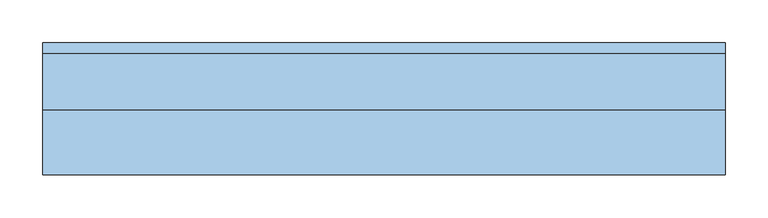
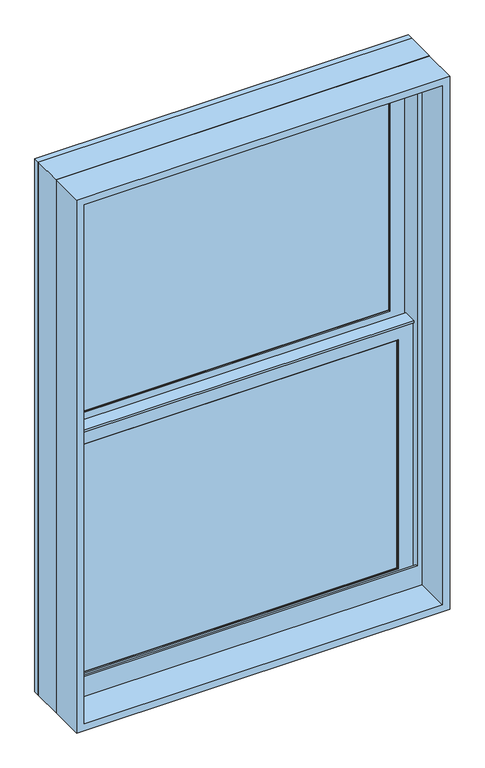
"""IFC4 building model written with IfcOpenShell, lengths in millimetres: window geometry, Window-Double_Hung-Marvin-Essential : ESDH2840."""

from ifc_helpers import new_model, si_unit, frame, origin, place, context, project, spatial, polyline, outline, extrude, faceted_brep, source, transform, mapped, element, save


def window_17e1d542(model_context):
    return source(origin(), model_context, "Body", "SolidModel", [
        extrude(outline(polyline([(123.825, 20.6375), (123.825, 15.875), (104.775, 15.875), (104.775, 20.6375), (123.825, 20.6375)])), frame((0.0, 0.0, 1289.05), z_axis=(0.0, 0.0, 1.0), x_axis=(1.0, 0.0, 0.0)), (0.0, 0.0, 1.0), 527.05),
        extrude(outline(polyline([(-104.775, 20.6375), (-104.775, 15.875), (-123.825, 15.875), (-123.825, 20.6375), (-104.775, 20.6375)])), frame((0.0, 0.0, 1289.05), z_axis=(0.0, 0.0, 1.0), x_axis=(1.0, 0.0, 0.0)), (0.0, 0.0, 1.0), 527.05),
        extrude(outline(polyline([(342.9, 20.6375), (342.9, 15.875), (-342.9, 15.875), (-342.9, 20.6375), (342.9, 20.6375)])), frame((0.0, 0.0, 1543.05), z_axis=(0.0, 0.0, 1.0), x_axis=(1.0, 0.0, 0.0)), (0.0, 0.0, 1.0), 19.05),
        extrude(outline(polyline([(-123.825, 46.83125), (-123.825, 51.59375), (-104.775, 51.59375), (-104.775, 46.83125), (-123.825, 46.83125)])), frame((0.0, 0.0, 1854.2), z_axis=(0.0, 0.0, 1.0), x_axis=(1.0, 0.0, 0.0)), (0.0, 0.0, 1.0), 527.05),
        extrude(outline(polyline([(104.775, 46.83125), (104.775, 51.59375), (123.825, 51.59375), (123.825, 46.83125), (104.775, 46.83125)])), frame((0.0, 0.0, 1854.2), z_axis=(0.0, 0.0, 1.0), x_axis=(1.0, 0.0, 0.0)), (0.0, 0.0, 1.0), 527.05),
        extrude(outline(polyline([(-342.9, 46.83125), (-342.9, 51.59375), (342.9, 51.59375), (342.9, 46.83125), (-342.9, 46.83125)])), frame((0.0, 0.0, 2108.2), z_axis=(0.0, 0.0, 1.0), x_axis=(1.0, 0.0, 0.0)), (0.0, 0.0, 1.0), 19.05),
        extrude(outline(polyline([(123.825, 20.6375), (104.775, 20.6375), (104.775, 25.4), (123.825, 25.4), (123.825, 20.6375)])), frame((0.0, 0.0, 1289.05), z_axis=(0.0, 0.0, 1.0), x_axis=(1.0, 0.0, 0.0)), (0.0, 0.0, 1.0), 527.05),
        extrude(outline(polyline([(-104.775, 20.6375), (-123.825, 20.6375), (-123.825, 25.4), (-104.775, 25.4), (-104.775, 20.6375)])), frame((0.0, 0.0, 1289.05), z_axis=(0.0, 0.0, 1.0), x_axis=(1.0, 0.0, 0.0)), (0.0, 0.0, 1.0), 527.05),
        extrude(outline(polyline([(342.9, 20.6375), (-342.9, 20.6375), (-342.9, 25.4), (342.9, 25.4), (342.9, 20.6375)])), frame((0.0, 0.0, 1543.05), z_axis=(0.0, 0.0, 1.0), x_axis=(1.0, 0.0, 0.0)), (0.0, 0.0, 1.0), 19.05),
        extrude(outline(polyline([(-123.825, 56.35625), (-104.775, 56.35625), (-104.775, 51.59375), (-123.825, 51.59375), (-123.825, 56.35625)])), frame((0.0, 0.0, 1854.2), z_axis=(0.0, 0.0, 1.0), x_axis=(1.0, 0.0, 0.0)), (0.0, 0.0, 1.0), 527.05),
        extrude(outline(polyline([(104.775, 56.35625), (123.825, 56.35625), (123.825, 51.59375), (104.775, 51.59375), (104.775, 56.35625)])), frame((0.0, 0.0, 1854.2), z_axis=(0.0, 0.0, 1.0), x_axis=(1.0, 0.0, 0.0)), (0.0, 0.0, 1.0), 527.05),
        extrude(outline(polyline([(-342.9, 56.35625), (342.9, 56.35625), (342.9, 51.59375), (-342.9, 51.59375), (-342.9, 56.35625)])), frame((0.0, 0.0, 2108.2), z_axis=(0.0, 0.0, 1.0), x_axis=(1.0, 0.0, 0.0)), (0.0, 0.0, 1.0), 19.05),
        faceted_brep([(-369.8875, 5.6780605, 1846.1351748), (-369.8875, 5.6780605, 1841.5), (369.8875, 5.6780605, 1841.5), (369.8875, 5.6780605, 1846.1351748), (-369.8875, 34.8118605, 1846.1351748), (369.8875, 34.8118605, 1846.1351748), (369.8875, 34.8118605, 1841.5), (-369.8875, 34.8118605, 1841.5), (-369.8875, 30.1625, 1841.5), (-369.8875, 30.1625, 1262.0625), (-369.8875, 8.9241104, 1262.0625), (-369.8875, 8.9241104, 1841.5), (369.8875, 8.9241104, 1841.5), (369.8875, 30.1625, 1841.5), (369.8875, 8.9241104, 1262.0625), (369.8875, 30.1625, 1262.0625), (-354.0034752, 11.90625, 1827.2034752), (-354.0034752, 30.1625, 1827.2034752), (354.0034752, 30.1625, 1827.2034752), (354.0034752, 11.90625, 1827.2034752), (-337.34375, 10.4662439, 1810.54375), (-337.34375, 11.90625, 1810.54375), (337.34375, 11.90625, 1810.54375), (337.34375, 10.4662439, 1810.54375), (338.8858834, 8.9241104, 1812.0858834), (-338.8858834, 8.9241104, 1812.0858834), (354.0034752, 30.1625, 1277.9465248), (354.0034752, 11.90625, 1277.9465248), (337.34375, 11.90625, 1294.60625), (337.34375, 10.4662439, 1294.60625), (338.8858834, 8.9241104, 1293.0641166), (-354.0034752, 30.1625, 1277.9465248), (-354.0034752, 11.90625, 1277.9465248), (-337.34375, 11.90625, 1294.60625), (-337.34375, 10.4662439, 1294.60625), (-338.8858834, 8.9241104, 1293.0641166)], [[[0, 1, 2, 3]], [[4, 5, 6, 7]], [[1, 0, 4, 7, 8, 9, 10, 11]], [[2, 1, 11, 12]], [[7, 6, 13, 8]], [[3, 2, 12, 14, 15, 13, 6, 5]], [[0, 3, 5, 4]], [[16, 17, 18, 19]], [[20, 21, 22, 23]], [[20, 23, 24, 25]], [[19, 18, 26, 27]], [[23, 22, 28, 29]], [[24, 23, 29, 30]], [[27, 26, 31, 32]], [[29, 28, 33, 34]], [[30, 29, 34, 35]], [[15, 14, 10, 9]], [[15, 9, 8, 13], [18, 17, 31, 26]], [[17, 16, 32, 31]], [[16, 19, 27, 32], [22, 21, 33, 28]], [[21, 20, 34, 33]], [[20, 25, 35, 34]], [[10, 14, 12, 11], [25, 24, 30, 35]]]),
        extrude(outline(polyline([(38.5955581, 1827.2125), (33.5778968, 1827.2125), (33.5778968, 1828.8), (39.9405976, 1828.8), (39.9405976, 1827.2125), (61.515625, 1827.2125), (47.6307501, 1823.8975159), (38.5955581, 1823.8975159), (38.5955581, 1827.2125)])), frame((-369.8875, 0.0, 0.0), z_axis=(1.0, 0.0, 0.0), x_axis=(0.0, 1.0, 0.0)), (0.0, 0.0, 1.0), 739.775),
        faceted_brep([(400.05, 0.0, 1231.9), (400.05, 0.0, 2438.4), (-400.05, 0.0, 2438.4), (-400.05, 0.0, 1231.9), (373.85625, 0.0, 1293.01875), (-373.85625, 0.0, 1293.01875), (-373.85625, 0.0, 2412.20625), (373.85625, 0.0, 2412.20625), (373.85625, 3.96875, 1231.9), (-373.85625, 3.96875, 1231.9), (-373.85625, 3.96875, 1293.01875), (373.85625, 3.96875, 1293.01875), (-400.05, 65.6828125, 1231.9), (-373.85625, 65.6828125, 1231.9), (373.85625, 65.6828125, 1231.9), (400.05, 65.6828125, 1231.9), (-400.05, 65.6828125, 2438.4), (400.05, 65.6828125, 2438.4), (373.85625, 65.6828125, 2412.20625), (-373.85625, 65.6828125, 2412.20625)], [[[0, 1, 2, 3], [4, 5, 6, 7]], [[8, 9, 10, 11]], [[5, 4, 11, 10]], [[0, 3, 12, 13, 9, 8, 14, 15]], [[13, 12, 16, 17, 15, 14, 18, 19]], [[13, 19, 6, 5, 10, 9]], [[7, 6, 19, 18]], [[18, 14, 8, 11, 4, 7]], [[1, 0, 15, 17]], [[2, 1, 17, 16]], [[3, 2, 16, 12]]]),
        faceted_brep([(373.85625, 30.1625, 1835.15), (372.26875, 30.1625, 1835.15), (372.26875, 30.1625, 1256.2544613), (373.85625, 30.1625, 1256.2544613), (-372.26875, 30.1625, 1835.15), (-373.85625, 30.1625, 1835.15), (-373.85625, 30.1625, 1256.2544613), (-372.26875, 30.1625, 1256.2544613), (372.26875, 63.5, 1835.15), (373.85625, 63.5, 1835.15), (373.85625, 63.5, 1249.7743077), (372.26875, 63.5, 1249.7743077), (-373.85625, 63.5, 1835.15), (-372.26875, 63.5, 1835.15), (-372.26875, 63.5, 1249.7743077), (-373.85625, 63.5, 1249.7743077), (385.1108932, 3.96875, 1261.3460105), (385.1108932, 3.96875, 1231.9), (385.1108932, 65.6828125, 1231.9), (385.1108932, 65.6828125, 1249.350012), (-385.1108932, 3.96875, 1231.9), (-385.1108932, 3.96875, 1261.3460105), (-385.1108932, 65.6828125, 1249.350012), (-385.1108932, 65.6828125, 1231.9), (385.1108932, 78.58125, 1246.8428097), (-385.1108932, 78.58125, 1246.8428097), (-383.0971252, 68.2348864, 1248.8539391), (-365.13135, 68.2348864, 1248.8539391), (-365.13135, 65.6828125, 1249.350012), (365.13135, 65.6828125, 1249.350012), (365.13135, 68.2348864, 1248.8539391), (383.0971252, 68.2348864, 1248.8539391), (-400.05, 65.6828125, 1231.9), (-400.05, 78.5948249, 1231.9), (400.05, 78.5948249, 1231.9), (400.05, 65.6828125, 1231.9), (-400.05, 78.58125, 2438.4), (400.05, 78.58125, 2438.4), (385.1108932, 78.58125, 2423.4608932), (-385.1108932, 78.58125, 2423.4608932), (-400.05, 65.6828125, 2438.4), (-383.0971252, 68.2348864, 2421.4471252), (383.0971252, 68.2348864, 2421.4471252), (365.13135, 68.2348864, 2403.48135), (-365.13135, 68.2348864, 2403.48135), (-365.13135, 65.6828125, 2403.48135), (365.13135, 65.6828125, 2403.48135), (400.05, 65.6828125, 2438.4)], [[[0, 1, 2, 3]], [[4, 5, 6, 7]], [[8, 9, 10, 11]], [[12, 13, 14, 15]], [[1, 8, 11, 2]], [[9, 0, 3, 10]], [[1, 0, 9, 8]], [[5, 4, 13, 12]], [[5, 12, 15, 6]], [[13, 4, 7, 14]], [[16, 17, 18, 19]], [[20, 21, 22, 23]], [[24, 25, 26, 27, 28, 22, 21, 16, 19, 29, 30, 31], [3, 2, 11, 10], [7, 6, 15, 14]], [[17, 16, 21, 20]], [[17, 20, 23, 32, 33, 34, 35, 18]], [[34, 33, 36, 37], [25, 24, 38, 39]], [[33, 32, 40, 36]], [[39, 41, 26, 25]], [[41, 42, 31, 30, 43, 44, 27, 26]], [[44, 45, 28, 27]], [[40, 32, 23, 22, 28, 45, 46, 29, 19, 18, 35, 47]], [[36, 40, 47, 37]], [[39, 38, 42, 41]], [[44, 43, 46, 45]], [[34, 37, 47, 35]], [[42, 38, 24, 31]], [[46, 43, 30, 29]]]),
        extrude(outline(polyline([(350.04375, 11.90625), (-350.04375, 11.90625), (-350.04375, 15.08125), (350.04375, 15.08125), (350.04375, 11.90625)])), frame((0.0, 0.0, 1281.90625), z_axis=(0.0, 0.0, 1.0), x_axis=(1.0, 0.0, 0.0)), (0.0, 0.0, 1.0), 541.3375),
        extrude(outline(polyline([(350.04375, 42.8625), (-350.04375, 42.8625), (-350.04375, 46.0375), (350.04375, 46.0375), (350.04375, 42.8625)])), frame((0.0, 0.0, 1847.05625), z_axis=(0.0, 0.0, 1.0), x_axis=(1.0, 0.0, 0.0)), (0.0, 0.0, 1.0), 541.3375),
        faceted_brep([(-337.34375, 31.194477, 1810.54375), (-338.8858834, 32.7366104, 1812.0858834), (338.8858834, 32.7366104, 1812.0858834), (337.34375, 31.194477, 1810.54375), (-337.34375, 30.1625, 1810.54375), (337.34375, 30.1625, 1810.54375), (-369.8875, 32.7366104, 1843.0875), (-369.8875, 30.1625, 1843.0875), (369.8875, 30.1625, 1843.0875), (369.8875, 32.7366104, 1843.0875), (338.8858834, 32.7366104, 1293.0641166), (337.34375, 31.194477, 1294.60625), (337.34375, 30.1625, 1294.60625), (369.8875, 30.1625, 1262.0625), (369.8875, 32.7366104, 1262.0625), (-338.8858834, 32.7366104, 1293.0641166), (-337.34375, 31.194477, 1294.60625), (-337.34375, 30.1625, 1294.60625), (-369.8875, 30.1625, 1262.0625), (-369.8875, 32.7366104, 1262.0625)], [[[0, 1, 2, 3]], [[4, 0, 3, 5]], [[6, 7, 8, 9]], [[3, 2, 10, 11]], [[5, 3, 11, 12]], [[9, 8, 13, 14]], [[11, 10, 15, 16]], [[12, 11, 16, 17]], [[14, 13, 18, 19]], [[9, 14, 19, 6], [1, 15, 10, 2]], [[16, 15, 1, 0]], [[17, 16, 0, 4]], [[7, 18, 13, 8], [5, 12, 17, 4]], [[19, 18, 7, 6]]]),
        faceted_brep([(-354.0034752, 42.8625, 2392.3534752), (-354.0034752, 61.11875, 2392.3534752), (354.0034752, 61.11875, 2392.3534752), (354.0034752, 42.8625, 2392.3534752), (-337.34375, 41.4224939, 2375.69375), (-337.34375, 42.8625, 2375.69375), (337.34375, 42.8625, 2375.69375), (337.34375, 41.4224939, 2375.69375), (-338.8858834, 39.8803604, 2377.2358834), (338.8858834, 39.8803604, 2377.2358834), (-369.8875, 61.11875, 2408.2375), (-369.8875, 39.8803604, 2408.2375), (369.8875, 39.8803604, 2408.2375), (369.8875, 61.11875, 2408.2375), (354.0034752, 61.11875, 1843.0965248), (354.0034752, 42.8625, 1843.0965248), (337.34375, 42.8625, 1859.75625), (337.34375, 41.4224939, 1859.75625), (338.8858834, 39.8803604, 1858.2141166), (369.8875, 39.8803604, 1827.2125), (369.8875, 61.11875, 1827.2125), (-354.0034752, 61.11875, 1843.0965248), (-354.0034752, 42.8625, 1843.0965248), (-337.34375, 42.8625, 1859.75625), (-337.34375, 41.4224939, 1859.75625), (-338.8858834, 39.8803604, 1858.2141166), (-369.8875, 39.8803604, 1827.2125), (-369.8875, 61.11875, 1827.2125)], [[[0, 1, 2, 3]], [[4, 5, 6, 7]], [[8, 4, 7, 9]], [[10, 11, 12, 13]], [[3, 2, 14, 15]], [[7, 6, 16, 17]], [[9, 7, 17, 18]], [[13, 12, 19, 20]], [[15, 14, 21, 22]], [[17, 16, 23, 24]], [[18, 17, 24, 25]], [[20, 19, 26, 27]], [[13, 20, 27, 10], [1, 21, 14, 2]], [[22, 21, 1, 0]], [[3, 15, 22, 0], [5, 23, 16, 6]], [[24, 23, 5, 4]], [[25, 24, 4, 8]], [[11, 26, 19, 12], [9, 18, 25, 8]], [[27, 26, 11, 10]]]),
        faceted_brep([(-369.8875, 61.11875, 1827.2125), (-369.8875, 63.6928604, 1827.2125), (369.8875, 63.6928604, 1827.2125), (369.8875, 61.11875, 1827.2125), (-337.34375, 62.150727, 1859.75625), (-337.34375, 61.11875, 1859.75625), (337.34375, 61.11875, 1859.75625), (337.34375, 62.150727, 1859.75625), (-338.8858834, 63.6928604, 1858.2141166), (338.8858834, 63.6928604, 1858.2141166), (369.8875, 63.6928604, 2408.2375), (369.8875, 61.11875, 2408.2375), (337.34375, 61.11875, 2375.69375), (337.34375, 62.150727, 2375.69375), (338.8858834, 63.6928604, 2377.2358834), (-369.8875, 63.6928604, 2408.2375), (-369.8875, 61.11875, 2408.2375), (-337.34375, 61.11875, 2375.69375), (-337.34375, 62.150727, 2375.69375), (-338.8858834, 63.6928604, 2377.2358834)], [[[0, 1, 2, 3]], [[4, 5, 6, 7]], [[8, 4, 7, 9]], [[3, 2, 10, 11]], [[7, 6, 12, 13]], [[9, 7, 13, 14]], [[11, 10, 15, 16]], [[13, 12, 17, 18]], [[14, 13, 18, 19]], [[16, 15, 1, 0]], [[3, 11, 16, 0], [5, 17, 12, 6]], [[18, 17, 5, 4]], [[19, 18, 4, 8]], [[1, 15, 10, 2], [9, 14, 19, 8]]]),
        extrude(outline(polyline([(350.04375, 26.19375), (-350.04375, 26.19375), (-350.04375, 30.1625), (350.04375, 30.1625), (350.04375, 26.19375)])), frame((0.0, 0.0, 1281.90625), z_axis=(0.0, 0.0, 1.0), x_axis=(1.0, 0.0, 0.0)), (0.0, 0.0, 1.0), 541.3375),
        extrude(outline(polyline([(350.04375, 57.15), (-350.04375, 57.15), (-350.04375, 61.11875), (350.04375, 61.11875), (350.04375, 57.15)])), frame((0.0, 0.0, 1847.05625), z_axis=(0.0, 0.0, 1.0), x_axis=(1.0, 0.0, 0.0)), (0.0, 0.0, 1.0), 541.3375),
        extrude(outline(polyline([(2438.4, 400.05), (2438.4, -400.05), (1231.9, -400.05), (1231.9, 400.05), (2438.4, 400.05)]), holes=[polyline([(2422.525, 384.175), (1247.775, 384.175), (1247.775, -384.175), (2422.525, -384.175), (2422.525, 384.175)])]), frame((0.0, -76.2, 0.0), z_axis=(0.0, 1.0, 0.0), x_axis=(0.0, 0.0, 1.0)), (0.0, 0.0, 1.0), 75.40625),
    ])


if __name__ == "__main__":
    model = new_model("IFC4")
    model_context = context("Model", 3, world=origin())
    ifc_project = project(units=[si_unit("LENGTHUNIT", "METRE", prefix="MILLI")], contexts=[model_context])
    site = spatial("IfcSite", under=ifc_project)
    building = spatial("IfcBuilding", under=site)
    placement = place(None, origin())
    window_shape = window_17e1d542(model_context)
    element("IfcWindow", 1, ObjectType="Window-Double_Hung-Marvin-Essential : ESDH2840", at=placement, inside=building, context=model_context, shape_type="MappedRepresentation", body=[
        mapped(window_shape, transform((0.0, 0.0, 0.0), x_axis=(1.0, 0.0, 0.0), y_axis=(0.0, 1.0, 0.0), z_axis=(0.0, 0.0, 1.0))),
    ])
    save(model, "model.ifc")

# Revit data of these elements
# Type "Window-Double_Hung-Marvin-Essential : ESDH2840"
#   Type Mark = "50"
#   Window Type = "Essential Double Hung"
#   Product data url = "https://bimobject.com/marvin-windows-and-doors/product/marvin-dhwau"
#   Product Guid = "c4a96547-874c-4385-91dc-a058adc19d98"
#   Frame = "All Ultrex"
#   Egress Window = "No"
#   URL = "www.marvin.com"
#   Model = "ESDH2840"
#   Manufacturer = "Marvin Windows and Doors"
#   Label Egress = ""
#   Glass Type = "IG Low E II with Argon"
#   Design Pressure = "DP50"
#   Description = "3248 DBHG"
#   Analytic Construction = "<None>"
#   Prairie Corner Width = 0' - 4"
#   Prairie Corner Height = 0' - 4"
#   Egress Width = 2' - 4 9/16"
#   Egress Height = 1' - 7 27/128"
#   Rough Width = 2' - 8"
#   Rough Height = 4' - 0"
#   Nominal Width = 2' - 8"
#   Nominal Height = 4' - 0"
#   Inset to Installation Flange [instance default] = 0' - 1"
#   Height = 3' - 11 1/2"
#   Egress Area = 3.8105 SF
#   Default Head Height = 8' - 0"
#   Width = 2' - 7 1/2"
#   Daylight Area = 7.49376 SF
#   DLO Width = 2' - 2 9/16"
#   DLO Height = 1' - 8 5/16"
#   Muntins Top Sash = yes
#   Lites Wide Top Sash = 3
#   Lites Wide Bottom Sash = 3
#   Lites High Top Sash = 2
#   Lites High Bottom Sash = 2
#   Lite Cut Prairie 9 = no
#   Lite Cut HV Grid = yes
#   Muntins Bottom Sash = yes
#   Label Visibility = no
#   Jamb Extension Visibility = yes
#   Edition number = 1
#   Interior Material = Ultrex-Marvin-Stonewhite
#   Glazing Material = Glass-Marvin-IG Low E II with Argon
#   Cladding Material = Ultrex-Marvin-Pebblegray
#   Wall Closure = (empty or 0)
#   Assembly Code = ""
# Element 1 (IfcWindow, "Window-Double_Hung-Marvin-Essential : ESDH2840")
#   Materials on its faces: "Ultrex-Marvin-Pebblegray", "Ultrex-Marvin-Stonewhite", "Glass-Marvin-IG Low E II with Argon"
# Materials
#   "Ultrex-Marvin-Stonewhite": class "Paint", colour RGB 250 251 245, transparency 0
#   "Glass-Marvin-IG Low E II with Argon": class "Glass", colour RGB 0 128 192, transparency 0.85
#   "Ultrex-Marvin-Pebblegray": class "Paint", colour RGB 189 185 173, transparency 0
